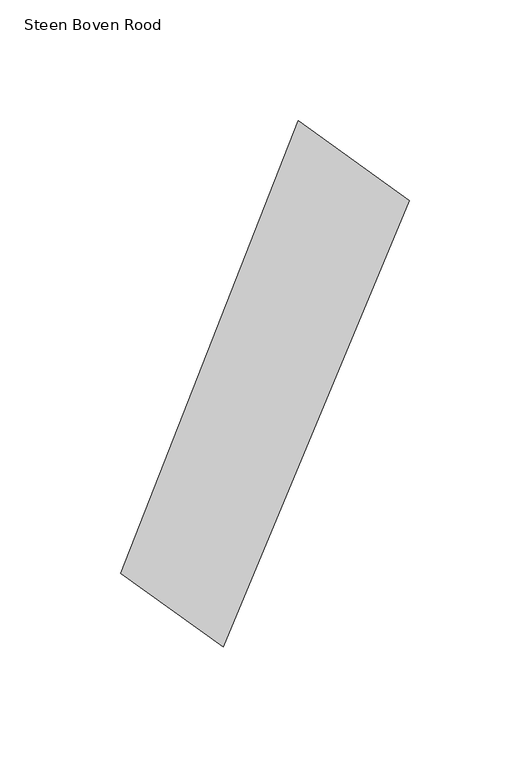
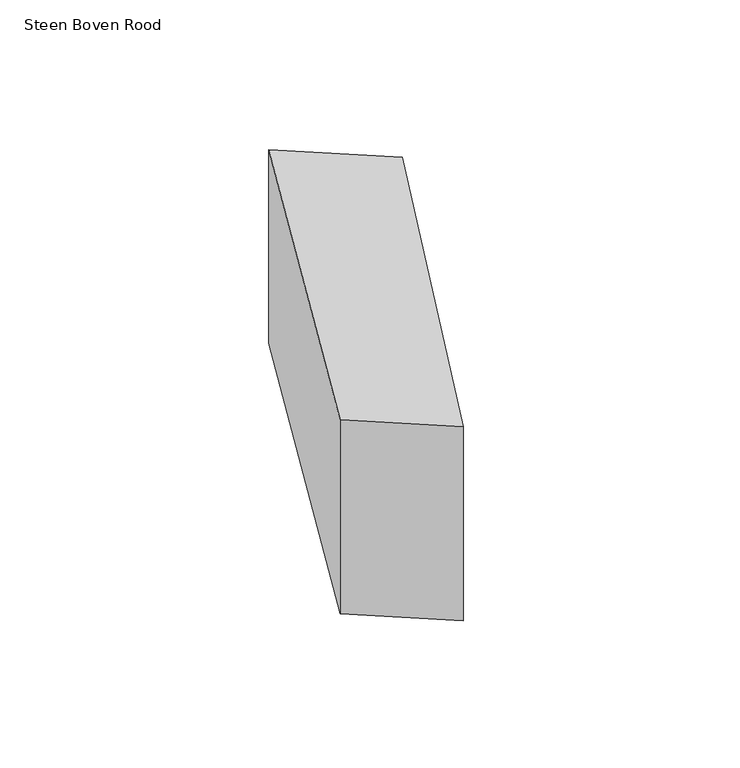
"""IFC4 building model written with IfcOpenShell, lengths in millimetres: proxy geometry, 00_GMA_steen_versie_4 : Steen Boven Rood."""

from ifc_helpers import new_model, si_unit, origin, origin_with_axes, place, context, project, spatial, polyline, outline, extrude, source, transform, mapped, element, save


def steen_boven_rood_4e10268b(model_context):
    return source(origin(), model_context, "Body", "SweptSolid", [
        extrude(outline(polyline([(140.9505476, 166.3193798), (63.9580448, -18.6724816), (21.4706832, 11.8665499), (94.950193, 199.41135), (140.9505476, 166.3193798)])), origin_with_axes(), (0.0, 0.0, 1.0), 100.0),
    ])


if __name__ == "__main__":
    model = new_model("IFC4")
    model_context = context("Model", 3, world=origin())
    ifc_project = project(units=[si_unit("LENGTHUNIT", "METRE", prefix="MILLI")], contexts=[model_context])
    site = spatial("IfcSite", under=ifc_project)
    building = spatial("IfcBuilding", under=site)
    placement = place(None, origin())
    steen_boven_rood_shape = steen_boven_rood_4e10268b(model_context)
    element("IfcBuildingElementProxy", 1, Name="00_GMA_steen_versie_4 : Steen Boven Rood", ObjectType="00_GMA_steen_versie_4 : Steen Boven Rood", at=placement, inside=building, context=model_context, shape_type="MappedRepresentation", body=[
        mapped(steen_boven_rood_shape, transform((0.0, 0.0, 0.0), x_axis=(1.0, 0.0, 0.0), y_axis=(0.0, 1.0, 0.0), z_axis=(0.0, 0.0, 1.0))),
    ])
    save(model, "model.ifc")

# Revit data of these elements
# Type "00_GMA_steen_versie_4 : Steen Boven Rood"
#   StootVoegHalfBoven [instance default] = 5 mm
#   StootVoegHalf [instance default] = 5 mm
#   StootVoegBreedteOnder = 10 mm
#   StootVoegBreedteBoven = 10 mm
#   Steendikte = 100 mm
#   LintVoegOnderHalf = 5 mm
#   LintVoegOnder = 10 mm
#   LintVoegBovenHalf = 0 mm
#   LintVoegBoven = 0 mm
#   materiaal = 21_steen_rood
#   MateriaalVoeg = none
#   Default Elevation = 0
# Element 1 (IfcBuildingElementProxy, "00_GMA_steen_versie_4 : Steen Boven Rood")
#   Materials on its faces: "21_steen_rood"
# Materials
#   "21_steen_rood": class "Unassigned", colour RGB 213 111 43, transparency 0, Cost = 0
